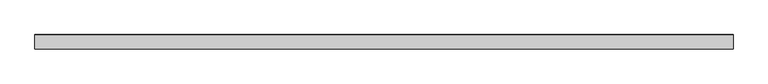
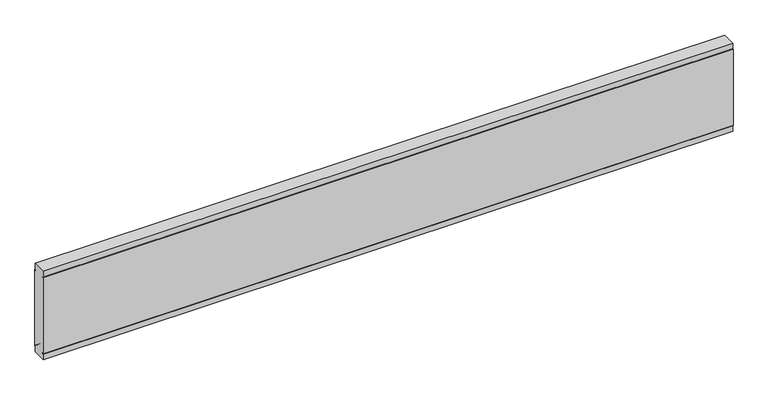
"""IFC4 building model written with IfcOpenShell, lengths in millimetres: proxy geometry, Generic Models 7:Generic Models 1:5:Generic Models 1:5 : Generic Models 7:Generic Models 1:337419:37 : Generic Models 7:Generic Models 1:5:Generic Models 1:5 : Generic Models 7:Generic Models 1:337419:311462."""

from ifc_helpers import new_model, si_unit, frame, origin, place, context, project, spatial, polyline, outline, extrude, source, transform, mapped, element, save


def generic_models_6b83ce22(model_context):
    return source(origin(), model_context, "Body", "SweptSolid", [
        extrude(outline(polyline([(-578799.0788841, 4893.9308169), (-578799.0788841, 3767.0723081), (-578812.2802009, 3778.1495282), (-578816.1067959, 3773.5891699), (-578801.8570091, 3761.632179), (-578801.8570091, 3679.428125), (-578996.3257591, 3679.428125), (-578996.3257591, 3761.632179), (-578982.0759722, 3773.5891699), (-578985.9025672, 3778.1495282), (-578999.1038841, 3767.0723081), (-578999.1038841, 4893.9308169), (-578985.9025672, 4882.8535968), (-578982.0759722, 4887.4139551), (-578996.3257591, 4899.370946), (-578996.3257591, 4981.575), (-578801.8570091, 4981.575), (-578801.8570091, 4899.370946), (-578816.1067959, 4887.4139551), (-578812.2802009, 4882.8535968), (-578799.0788841, 4893.9308169)])), frame((793322.7632437, 0.0, 0.0), z_axis=(1.0, 0.0, 0.0), x_axis=(0.0, 1.0, 0.0)), (0.0, 0.0, 1.0), 9631.124044),
    ])


if __name__ == "__main__":
    model = new_model("IFC4")
    model_context = context("Model", 3, world=origin())
    ifc_project = project(units=[si_unit("LENGTHUNIT", "METRE", prefix="MILLI")], contexts=[model_context])
    site = spatial("IfcSite", under=ifc_project)
    building = spatial("IfcBuilding", under=site)
    placement = place(None, origin())
    generic_models_shape = generic_models_6b83ce22(model_context)
    element("IfcBuildingElementProxy", 1, Name="Generic Models 7:Generic Models 1:5:Generic Models 1:5 : Generic Models 7:Generic Models 1:337419:37 : Generic Models 7:Generic Models 1:5:Generic Models 1:5 : Generic Models 7:Generic Models 1:337419:311462", ObjectType="Generic Models 7:Generic Models 1:5:Generic Models 1:5 : Generic Models 7:Generic Models 1:337419:37 : Generic Models 7:Generic Models 1:5:Generic Models 1:5 : Generic Models 7:Generic Models 1:337419:311462", at=placement, inside=building, context=model_context, shape_type="MappedRepresentation", body=[
        mapped(generic_models_shape, transform((0.0, 0.0, 0.0), x_axis=(1.0, 0.0, 0.0), y_axis=(0.0, 1.0, 0.0), z_axis=(0.0, 0.0, 1.0))),
    ])
    save(model, "model.ifc")

# Revit data of these elements
# Type "Generic Models 7:Generic Models 1:5:Generic Models 1:5 : Generic Models 7:Generic Models 1:337419:37 : Generic Models 7:Generic Models 1:5:Generic Models 1:5 : Generic Models 7:Generic Models 1:337419:311462"
#   NameOverride = "Generic Models 7:Generic Models 1:5:Generic Models 1:5 : Generic Models 7:Generic Models 1:337419:311462"
#   ObjectTypeOverride = "Generic Models 1:5 : Generic Models 7:Generic Models 1:337419"
#   Reference = "Generic Models 1"
#   Tag = "311462"
# Element 1 (IfcBuildingElementProxy, "Generic Models 7:Generic Models 1:5:Generic Models 1:5 : Generic Models 7:Generic Models 1:337419:37 : Generic Models 7:Generic Models 1:5:Generic Models 1:5 : Generic Models 7:Generic Models 1:337419:311462")
#   Materials on its faces: "SIMPLE SAVER INSULATION WITH LINER - COLOR: BLACK"
# Materials
#   "SIMPLE SAVER INSULATION WITH LINER - COLOR: BLACK": class "Unassigned", colour RGB 158 92 175, transparency 0, Cost = 0
